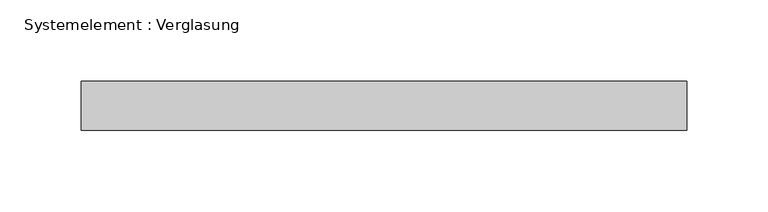
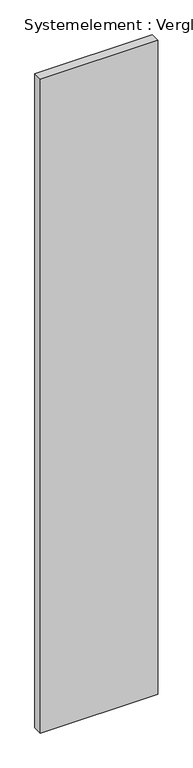
"""IFC4 building model written with IfcOpenShell, lengths in millimetres: plate geometry, Systemelement : Verglasung."""

from ifc_helpers import new_model, si_unit, origin, origin_with_axes, place, context, project, spatial, polyline, outline, extrude, source, transform, mapped, element, save


def systemelement_verglasung_543c2645(model_context):
    return source(origin(), model_context, "Body", "SweptSolid", [
        extrude(outline(polyline([(186.2499998, -15.0), (-186.2499998, -15.0), (-186.2499998, 15.0), (186.2499998, 15.0), (186.2499998, -15.0)])), origin_with_axes(), (0.0, 0.0, 1.0), 2190.0),
    ])


if __name__ == "__main__":
    model = new_model("IFC4")
    model_context = context("Model", 3, world=origin())
    ifc_project = project(units=[si_unit("LENGTHUNIT", "METRE", prefix="MILLI")], contexts=[model_context])
    site = spatial("IfcSite", under=ifc_project)
    building = spatial("IfcBuilding", under=site)
    placement = place(None, origin())
    systemelement_verglasung_shape = systemelement_verglasung_543c2645(model_context)
    element("IfcPlate", 1, ObjectType="Systemelement : Verglasung", at=placement, inside=building, context=model_context, shape_type="MappedRepresentation", body=[
        mapped(systemelement_verglasung_shape, transform((0.0, 0.0, 0.0), x_axis=(1.0, 0.0, 0.0), y_axis=(0.0, 1.0, 0.0), z_axis=(0.0, 0.0, 1.0))),
    ])
    save(model, "model.ifc")

# Revit data of these elements
# Type "Systemelement : Verglasung"
#   Construction Type Id = "GSP4R"
#   Analytic Construction = "1/8 Zoll Pilkington-Verglasung einfach"
#   Visual Light Transmittance = 0.9
#   Solar Heat Gain Coefficient = 0.86
#   Heat Transfer Coefficient (U) = 6.7069 W/(m²·K)
# Element 1 (IfcPlate, "Systemelement : Verglasung")
#   Materials on its faces: "Glas"
# Materials
#   "Glas": class "Glas", colour RGB 0 0 255, transparency 0.75, Comments = "Render-Darstellung nicht aktualisiert ", Cost = 0
